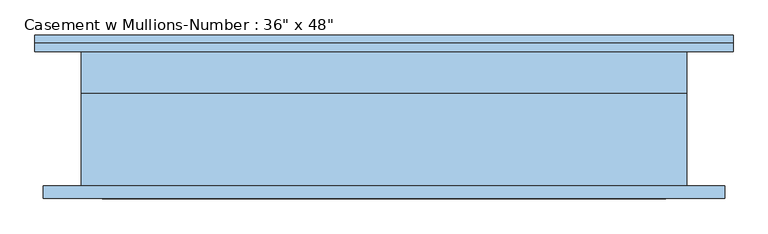
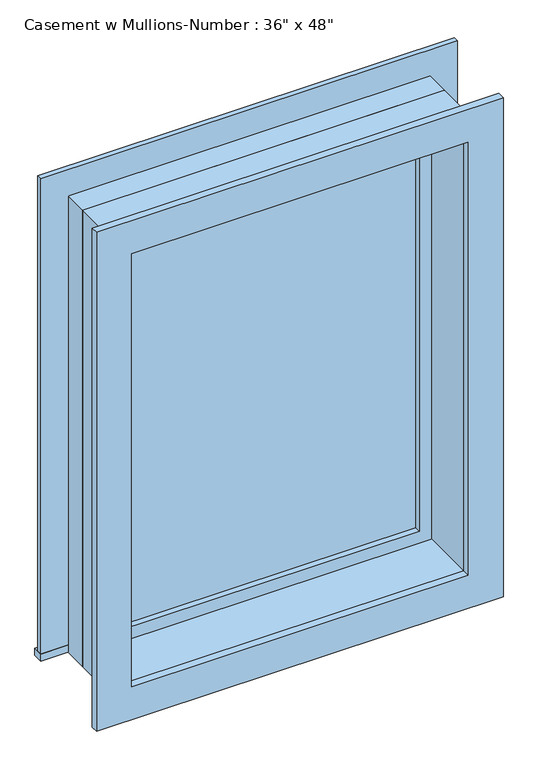
"""IFC4 building model written with IfcOpenShell, lengths in millimetres: window geometry."""

from ifc_helpers import new_model, si_unit, frame, origin, place, context, project, spatial, polyline, outline, extrude, source, transform, mapped, element, save


def window_0245c73a(model_context):
    return source(origin(), model_context, "Body", "SweptSolid", [
        extrude(outline(polyline([(-527.05, 127.0), (527.05, 127.0), (527.05, 101.6), (-527.05, 101.6), (-527.05, 127.0)])), frame((0.0, 0.0, 914.4), z_axis=(0.0, 0.0, 1.0), x_axis=(1.0, 0.0, 0.0)), (0.0, 0.0, 1.0), 19.05),
        extrude(outline(polyline([(2114.55, -438.15), (2114.55, 438.15), (933.45, 438.15), (933.45, 527.05), (2203.45, 527.05), (2203.45, -527.05), (933.45, -527.05), (933.45, -438.15), (2114.55, -438.15)])), frame((0.0, 101.6, 0.0), z_axis=(0.0, 1.0, 0.0), x_axis=(0.0, 0.0, 1.0)), (0.0, 0.0, 1.0), 12.7),
        extrude(outline(polyline([(-393.7, 66.675), (393.7, 66.675), (393.7, 53.975), (-393.7, 53.975), (-393.7, 66.675)])), frame((0.0, 0.0, 977.9), z_axis=(0.0, 0.0, 1.0), x_axis=(1.0, 0.0, 0.0)), (0.0, 0.0, 1.0), 1092.2),
        extrude(outline(polyline([(2190.75, 514.35), (2190.75, -514.35), (857.25, -514.35), (857.25, 514.35), (2190.75, 514.35)]), holes=[polyline([(2101.85, 425.45), (946.15, 425.45), (946.15, -425.45), (2101.85, -425.45), (2101.85, 425.45)])]), frame((0.0, -120.65, 0.0), z_axis=(0.0, 1.0, 0.0), x_axis=(0.0, 0.0, 1.0)), (0.0, 0.0, 1.0), 19.05),
        extrude(outline(polyline([(2114.55, -438.15), (933.45, -438.15), (933.45, 438.15), (2114.55, 438.15), (2114.55, -438.15)]), holes=[polyline([(2070.1, 393.7), (977.9, 393.7), (977.9, -393.7), (2070.1, -393.7), (2070.1, 393.7)])]), frame((0.0, 38.1, 0.0), z_axis=(0.0, 1.0, 0.0), x_axis=(0.0, 0.0, 1.0)), (0.0, 0.0, 1.0), 44.45),
        extrude(outline(polyline([(2133.6, -457.2), (914.4, -457.2), (914.4, 457.2), (2133.6, 457.2), (2133.6, -457.2)]), holes=[polyline([(2101.85, -425.45), (2101.85, 425.45), (946.15, 425.45), (946.15, -425.45), (2101.85, -425.45)])]), frame((0.0, -101.6, 0.0), z_axis=(0.0, 1.0, 0.0), x_axis=(0.0, 0.0, 1.0)), (0.0, 0.0, 1.0), 139.7),
        extrude(outline(polyline([(2133.6, 457.2), (2133.6, -457.2), (914.4, -457.2), (914.4, 457.2), (2133.6, 457.2)]), holes=[polyline([(2114.55, 438.15), (933.45, 438.15), (933.45, -438.15), (2114.55, -438.15), (2114.55, 438.15)])]), frame((0.0, 38.1, 0.0), z_axis=(0.0, 1.0, 0.0), x_axis=(0.0, 0.0, 1.0)), (0.0, 0.0, 1.0), 63.5),
    ])


if __name__ == "__main__":
    model = new_model("IFC4")
    model_context = context("Model", 3, world=origin())
    ifc_project = project(units=[si_unit("LENGTHUNIT", "METRE", prefix="MILLI")], contexts=[model_context])
    site = spatial("IfcSite", under=ifc_project)
    building = spatial("IfcBuilding", under=site)
    placement = place(None, origin())
    window_shape = window_0245c73a(model_context)
    element("IfcWindow", 1, ObjectType="Casement w Mullions-Number : 36\" x 48\"", at=placement, inside=building, context=model_context, shape_type="MappedRepresentation", body=[
        mapped(window_shape, transform((0.0, 0.0, 0.0), x_axis=(1.0, 0.0, 0.0), y_axis=(0.0, 1.0, 0.0), z_axis=(0.0, 0.0, 1.0))),
    ])
    save(model, "model.ifc")

# Revit data of these elements
# Project information
#   Organization Name = "G3B Press"
#   Organization Description = "Paul F. Aubin Cosulting Services, Inc."
#   Building Name = "Revit Essentials for Architecture"
#   Author = "Paul F. Aubin"
#   Author Website = "https://www.paulaubin.com"
#   Copyright = "Copyright © 2020 Paul F Aubin, all rights reserved"
#   Project Issue Date = "8/1/2020"
#   Project Status = "Schematic Design"
#   Client Name = "Rendering and Presentation"
#   Project Address = "567 Grove ST\nAnytown, IL 60000"
#   Project Name = "18 Pavilion"
#   Project Number = "2020.01A"
# Type "Casement w Mullions-Number : 36\" x 48\""
#   Type Mark = "18"
#   Assembly Code = "B2020100"
#   MWidth = 2.583333 ft
#   MHeight = 3.583333 ft
#   Height = 4.00 ft
#   Default Sill Height = 3.00 ft
#   Trim Projection - Ext. = 0.041667 ft
#   Trim Projection - Int. = 0.0625 ft
#   Trim Width - Exterior = 0.291667 ft
#   Trim Width - Interior = 0.291667 ft
#   Width = 3.00 ft
#   Window Inset = 0.0625 ft
#   Vertical Lites = 4
#   Trim Visible [instance default] = yes
#   Mullion Visible [instance default] = yes
#   Horizontal Lites = 4
#   Glass Pane Material = Glass, Clear Glazing
#   Sash Material = Maple - Semigloss
#   Trim Exterior Material = Clad - White
#   Trim Interior Material = Maple - Semigloss
#   Wall Closure = (empty or 0)
# Element 1 (IfcWindow, "Casement w Mullions-Number : 36\" x 48\"")
#   Materials on its faces: "Maple - Semigloss", "Clad - White", "Glass, Clear Glazing"
# Materials
#   "Glass, Clear Glazing": class "Glass", colour RGB 245 245 243, transparency 1, Description = "Clear glazing", Cost = 0
#   "Maple - Semigloss": class "Wood", colour RGB 196 161 118, transparency 0, Description = "Acer Saccharum", Cost = 0
#   "Clad - White": class "Wood", colour RGB 245 245 243, transparency 0, Cost = 0
